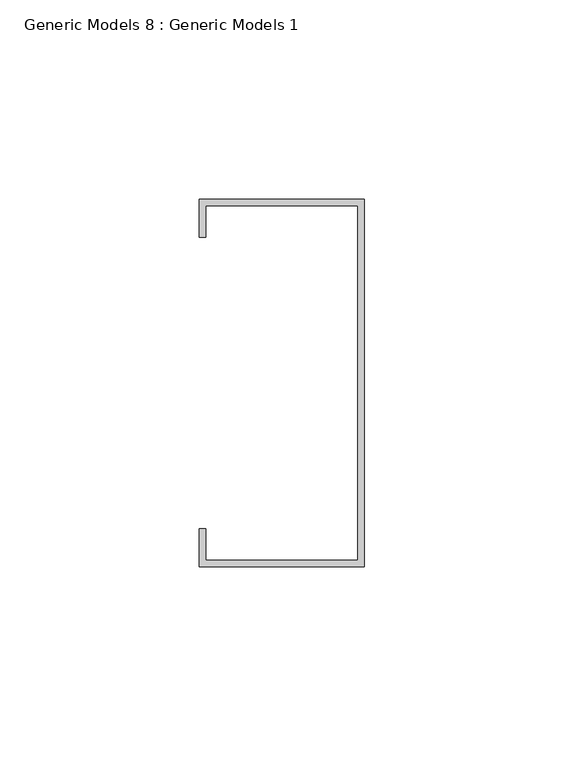
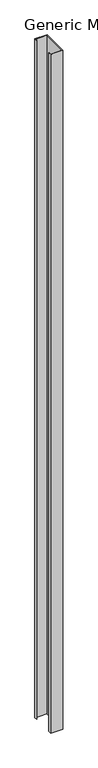
"""IFC4 building model written with IfcOpenShell, lengths in millimetres: proxy geometry, Generic Models 8 : Generic Models 1."""

from ifc_helpers import new_model, si_unit, frame, origin, place, context, project, spatial, polyline, outline, extrude, source, transform, mapped, element, save


def generic_models_8_generic_models_1_73c74f16(model_context):
    return source(origin(), model_context, "Body", "SweptSolid", [
        extrude(outline(polyline([(13691.4842846, 5685.6032424), (13691.4842846, 5593.5282424), (13650.2092846, 5593.5282424), (13650.2092846, 5603.0532424), (13651.7967846, 5603.0532424), (13651.7967846, 5595.1157424), (13689.8967846, 5595.1157424), (13689.8967846, 5684.0157424), (13651.7967846, 5684.0157424), (13651.7967846, 5676.0782424), (13650.2092846, 5676.0782424), (13650.2092846, 5685.6032424), (13691.4842846, 5685.6032424)])), frame((0.0, 0.0, 450.7860265), z_axis=(0.0, 0.0, 1.0), x_axis=(1.0, 0.0, 0.0)), (0.0, 0.0, 1.0), 2438.4),
    ])


if __name__ == "__main__":
    model = new_model("IFC4")
    model_context = context("Model", 3, world=origin())
    ifc_project = project(units=[si_unit("LENGTHUNIT", "METRE", prefix="MILLI")], contexts=[model_context])
    site = spatial("IfcSite", under=ifc_project)
    building = spatial("IfcBuilding", under=site)
    placement = place(None, origin())
    generic_models_8_generic_models_1_shape = generic_models_8_generic_models_1_73c74f16(model_context)
    element("IfcBuildingElementProxy", 1, Name="Generic Models 8 : Generic Models 1", ObjectType="Generic Models 8 : Generic Models 1", at=placement, inside=building, context=model_context, shape_type="MappedRepresentation", body=[
        mapped(generic_models_8_generic_models_1_shape, transform((0.0, 0.0, 0.0), x_axis=(1.0, 0.0, 0.0), y_axis=(0.0, 1.0, 0.0), z_axis=(0.0, 0.0, 1.0))),
    ])
    save(model, "model.ifc")

# Revit data of these elements
# Element 1 (IfcBuildingElementProxy, "Generic Models 8 : Generic Models 1")
#   Materials on its faces: "METAL STUDS"
# Materials
#   "METAL STUDS": class "Unassigned", colour RGB 210 209 208, transparency 0, Keynote = "M05121300.02", Cost = 0
